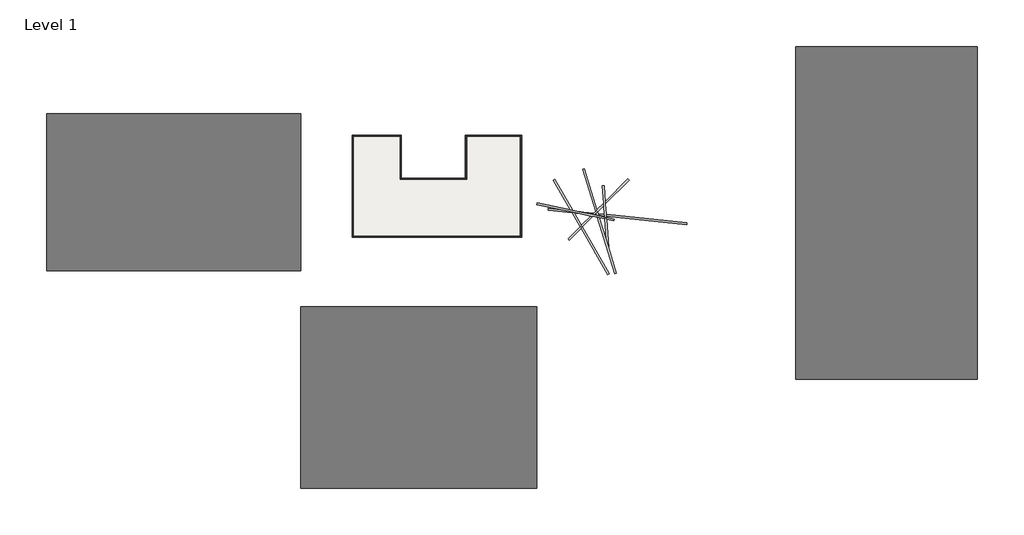
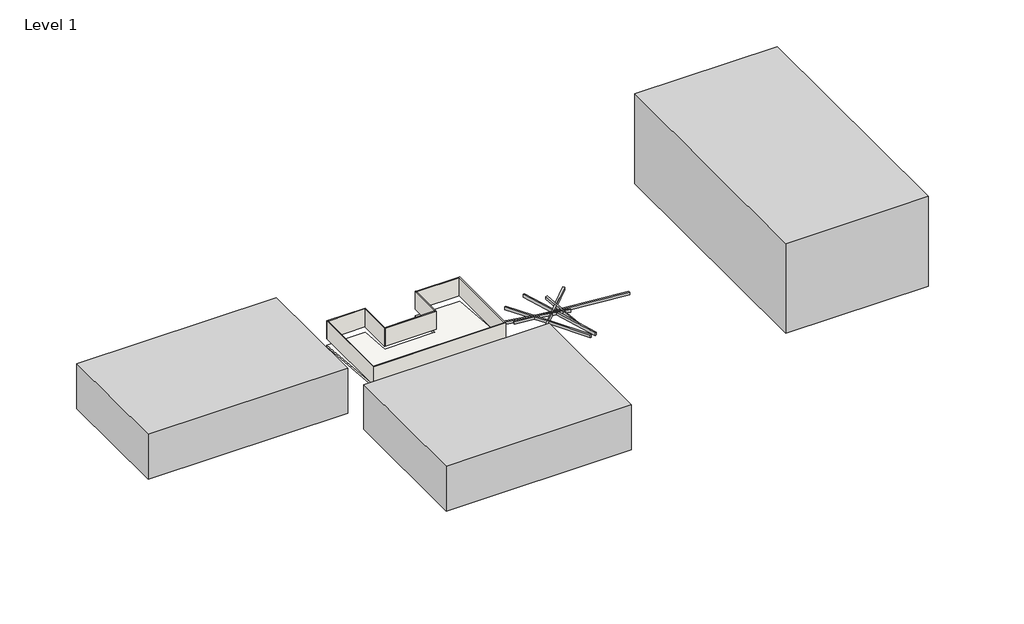
# One storey: 8 walls, 6 beams, 1 proxy, 1 slab.
"""IFC4 building model written with IfcOpenShell, lengths in millimetres."""

from ifc_helpers import new_model, si_unit, frame, origin, origin_with_axes, place, context, project, spatial, polyline, outline, extrude, faceted_brep, element, save

model = new_model("IFC4")

# Units and contexts
model_context = context("Model", 3, world=origin())
ifc_project = project(units=[si_unit("LENGTHUNIT", "METRE", prefix="MILLI")], contexts=[model_context])

# Site, building, storey
site = spatial("IfcSite", under=ifc_project)
building = spatial("IfcBuilding", under=site)
storey = spatial("IfcBuildingStorey", under=building, Name="Level 1", Elevation=0.0)

# Beams
placement = place(None, origin())
element("IfcBeam", 1, ObjectType="M_Concrete-Rectangular Beam : 300 x 600mm", at=placement, inside=storey, context=model_context, shape_type="Brep", body=[
    faceted_brep([(23275.0749275, 1168.1694607, 0.0), (23574.3441426, 1189.0964028, 0.0), (23574.3441426, 1189.0964028, -600.0), (23275.0749275, 1168.1694607, -600.0), (23478.0913387, -1735.1004802, 0.0), (23505.8198089, -2131.6360787, 0.0), (23605.6683255, -3559.5363899, 0.0), (23626.9180994, -3863.422315, 0.0), (23638.1515547, -4024.0682104, 0.0), (23659.9218408, -4335.397806, 0.0), (23902.8471924, -7809.3921842, 0.0), (24292.7609524, -9084.7426271, 0.0), (23965.19176, -4400.2849304, 0.0), (23943.4214739, -4088.9553348, 0.0), (23929.877299, -3895.26461, 0.0), (23908.6275251, -3591.3786849, 0.0), (23786.8975108, -1850.5583769, 0.0), (23759.1690405, -1454.0227784, 0.0), (24292.7609524, -9084.7426271, -600.0), (23965.19176, -4400.2849304, -600.0), (23943.4214739, -4088.9553348, -600.0), (23929.877299, -3895.26461, -600.0), (23908.6275251, -3591.3786849, -600.0), (23786.8975108, -1850.5583769, -600.0), (23759.1690405, -1454.0227784, -600.0), (23902.8471924, -7809.3921842, -600.0), (23659.9218408, -4335.397806, -600.0), (23638.1515547, -4024.0682104, -600.0), (23626.9180994, -3863.422315, -600.0), (23605.6683255, -3559.5363899, -600.0), (23505.8198089, -2131.6360787, -600.0), (23478.0913387, -1735.1004802, -600.0)], [[[0, 1, 2, 3]], [[1, 0, 4, 5, 6, 7, 8, 9, 10, 11, 12, 13, 14, 15, 16, 17]], [[2, 1, 17, 16, 15, 14, 13, 12, 11, 18, 19, 20, 21, 22, 23, 24]], [[3, 2, 24, 23, 22, 21, 20, 19, 18, 25, 26, 27, 28, 29, 30, 31]], [[0, 3, 31, 30, 29, 28, 27, 26, 25, 10, 9, 8, 7, 6, 5, 4]], [[11, 10, 25, 18]]]),
])
element("IfcBeam", 2, ObjectType="M_Concrete-Rectangular Beam : 300 x 600mm", at=placement, inside=storey, context=model_context, shape_type="Brep", body=[
    faceted_brep([(12450.0596621, -1952.6680445, 0.0), (12512.4331694, -1659.2237643, 0.0), (12512.4331694, -1659.2237643, -600.0), (12450.0596621, -1952.6680445, -600.0), (16492.4721668, -2811.9093474, 0.0), (19299.7867589, -3408.6224846, 0.0), (21365.4904585, -3847.7013604, 0.0), (21715.3826467, -3922.0732409, 0.0), (22448.2953753, -4077.8586505, 0.0), (22783.8060868, -4149.1736537, 0.0), (23659.9218408, -4335.397806, 0.0), (23638.1515547, -4024.0682104, 0.0), (22683.5207734, -3821.1551739, 0.0), (22348.0100619, -3749.8401706, 0.0), (22154.0960952, -3708.6224846, 0.0), (21968.3210977, -3669.1347899, 0.0), (21618.4289095, -3594.7629094, 0.0), (19346.7815031, -3111.9093474, 0.0), (18380.9429058, -2906.614016, 0.0), (17986.074678, -2822.6821832, 0.0), (23638.1515547, -4024.0682104, -600.0), (22683.5207734, -3821.1551739, -600.0), (22348.0100619, -3749.8401706, -600.0), (22154.0960952, -3708.6224846, -600.0), (21968.3210977, -3669.1347899, -600.0), (21618.4289095, -3594.7629094, -600.0), (19346.7815031, -3111.9093474, -600.0), (18380.9429058, -2906.614016, -600.0), (17986.074678, -2822.6821832, -600.0), (23659.9218408, -4335.397806, -600.0), (22783.8060868, -4149.1736537, -600.0), (22448.2953753, -4077.8586505, -600.0), (21715.3826467, -3922.0732409, -600.0), (21365.4904585, -3847.7013604, -600.0), (19299.7867589, -3408.6224846, -600.0), (16492.4721668, -2811.9093474, -600.0)], [[[0, 1, 2, 3]], [[1, 0, 4, 5, 6, 7, 8, 9, 10, 11, 12, 13, 14, 15, 16, 17, 18, 19]], [[2, 1, 19, 18, 17, 16, 15, 14, 13, 12, 11, 20, 21, 22, 23, 24, 25, 26, 27, 28]], [[3, 2, 28, 27, 26, 25, 24, 23, 22, 21, 20, 29, 30, 31, 32, 33, 34, 35]], [[0, 3, 35, 34, 33, 32, 31, 30, 29, 10, 9, 8, 7, 6, 5, 4]], [[11, 10, 29, 20]]]),
    faceted_brep([(25165.9784716, -4655.5200252, 0.0), (25165.9784716, -4655.5200252, -600.0), (25228.3519789, -4362.0757449, -600.0), (25228.3519789, -4362.0757449, 0.0), (23965.19176, -4400.2849304, 0.0), (23943.4214739, -4088.9553348, 0.0), (23943.4214739, -4088.9553348, -600.0), (23965.19176, -4400.2849304, -600.0)], [[[0, 1, 2, 3]], [[4, 5, 6, 7]], [[0, 3, 5, 4]], [[3, 2, 6, 5]], [[2, 1, 7, 6]], [[1, 0, 4, 7]]]),
])
element("IfcBeam", 3, ObjectType="M_Concrete-Rectangular Beam : 300 x 600mm", at=placement, inside=storey, context=model_context, shape_type="Brep", body=[
    faceted_brep([(17813.0913686, -7824.3645191, 0.0), (17600.9593342, -7612.2324847, 0.0), (17600.9593342, -7612.2324847, -600.0), (17813.0913686, -7824.3645191, -600.0), (19753.5011889, -5883.9546987, 0.0), (19973.1164312, -5664.3394565, 0.0), (21715.3826467, -3922.0732409, 0.0), (21365.4904585, -3847.7013604, 0.0), (19817.8250041, -5395.3668148, 0.0), (19598.2097619, -5614.9820571, 0.0), (21365.4904585, -3847.7013604, -600.0), (19817.8250041, -5395.3668148, -600.0), (19598.2097619, -5614.9820571, -600.0), (21715.3826467, -3922.0732409, -600.0), (19973.1164312, -5664.3394565, -600.0), (19753.5011889, -5883.9546987, -600.0)], [[[0, 1, 2, 3]], [[1, 0, 4, 5, 6, 7, 8, 9]], [[2, 1, 9, 8, 7, 10, 11, 12]], [[3, 2, 12, 11, 10, 13, 14, 15]], [[0, 3, 15, 14, 13, 6, 5, 4]], [[7, 6, 13, 10]]]),
    faceted_brep([(27712.5863052, 2075.1304175, 0.0), (27712.5863052, 2075.1304175, -600.0), (27500.4542708, 2287.2624519, -600.0), (27500.4542708, 2287.2624519, 0.0), (23786.8975108, -1850.5583769, 0.0), (23759.1690405, -1454.0227784, 0.0), (23759.1690405, -1454.0227784, -600.0), (23786.8975108, -1850.5583769, -600.0)], [[[0, 1, 2, 3]], [[4, 5, 6, 7]], [[0, 3, 5, 4]], [[3, 2, 6, 5]], [[2, 1, 7, 6]], [[1, 0, 4, 7]]]),
    faceted_brep([(23478.0913387, -1735.1004802, 0.0), (23505.8198089, -2131.6360787, 0.0), (23505.8198089, -2131.6360787, -600.0), (23478.0913387, -1735.1004802, -600.0), (21968.3210977, -3669.1347899, 0.0), (21618.4289095, -3594.7629094, 0.0), (21618.4289095, -3594.7629094, -600.0), (21968.3210977, -3669.1347899, -600.0), (22381.1258552, -2832.0659638, 0.0), (22140.8714663, -3072.3203527, 0.0), (21839.3074392, -3373.8843798, 0.0), (22223.2206079, -3414.2352798, 0.0), (22240.2108972, -3397.2449905, 0.0), (22480.4652861, -3156.9906016, 0.0), (22381.1258552, -2832.0659638, -600.0), (22140.8714663, -3072.3203527, -600.0), (21839.3074392, -3373.8843798, -600.0), (22480.4652861, -3156.9906016, -600.0), (22240.2108972, -3397.2449905, -600.0), (22223.2206079, -3414.2352798, -600.0)], [[[0, 1, 2, 3]], [[4, 5, 6, 7]], [[1, 0, 8, 9, 10, 5, 4, 11, 12, 13]], [[0, 3, 14, 15, 16, 6, 5, 10, 9, 8]], [[3, 2, 17, 18, 19, 7, 6, 16, 15, 14]], [[2, 1, 13, 12, 11, 4, 7, 19, 18, 17]]]),
])
element("IfcBeam", 4, ObjectType="M_Concrete-Rectangular Beam : 300 x 600mm", at=placement, inside=storey, context=model_context, shape_type="Brep", body=[
    faceted_brep([(25575.5456711, -13280.5423831, 0.0), (25288.6542443, -13368.2538946, 0.0), (25288.6542443, -13368.2538946, -600.0), (25575.5456711, -13280.5423831, -600.0), (24292.7609524, -9084.7426271, 0.0), (23902.8471924, -7809.3921842, 0.0), (22783.8060868, -4149.1736537, 0.0), (22448.2953753, -4077.8586505, 0.0), (22448.2953753, -4077.8586505, -600.0), (22783.8060868, -4149.1736537, -600.0), (23902.8471924, -7809.3921842, -600.0), (24292.7609524, -9084.7426271, -600.0)], [[[0, 1, 2, 3]], [[1, 0, 4, 5, 6, 7]], [[2, 1, 7, 8]], [[3, 2, 8, 9, 10, 11]], [[0, 3, 11, 10, 9, 6, 5, 4]], [[7, 6, 9, 8]]]),
    faceted_brep([(20312.8549861, 3932.9432242, 0.0), (20312.8549861, 3932.9432242, -600.0), (20025.9635593, 3845.2317128, -600.0), (20025.9635593, 3845.2317128, 0.0), (22381.1258552, -2832.0659638, 0.0), (22140.8714663, -3072.3203527, 0.0), (22140.8714663, -3072.3203527, -600.0), (22381.1258552, -2832.0659638, -600.0)], [[[0, 1, 2, 3]], [[4, 5, 6, 7]], [[0, 3, 5, 4]], [[3, 2, 6, 5]], [[2, 1, 7, 6]], [[1, 0, 4, 7]]]),
    faceted_brep([(22683.5207734, -3821.1551739, 0.0), (22348.0100619, -3749.8401706, 0.0), (22348.0100619, -3749.8401706, -600.0), (22683.5207734, -3821.1551739, -600.0), (22665.5509582, -3762.3785569, 0.0), (22570.2646476, -3450.7110782, 0.0), (22480.4652861, -3156.9906016, 0.0), (22240.2108972, -3397.2449905, 0.0), (22246.1418931, -3416.6444039, 0.0), (22341.4282037, -3728.3118826, 0.0), (22240.2108972, -3397.2449905, -600.0), (22246.1418931, -3416.6444039, -600.0), (22341.4282037, -3728.3118826, -600.0), (22480.4652861, -3156.9906016, -600.0), (22570.2646476, -3450.7110782, -600.0), (22665.5509582, -3762.3785569, -600.0)], [[[0, 1, 2, 3]], [[1, 0, 4, 5, 6, 7, 8, 9]], [[2, 1, 9, 8, 7, 10, 11, 12]], [[3, 2, 12, 11, 10, 13, 14, 15]], [[0, 3, 15, 14, 13, 6, 5, 4]], [[7, 6, 13, 10]]]),
])
element("IfcBeam", 5, ObjectType="M_Concrete-Rectangular Beam : 300 x 600mm", at=placement, inside=storey, context=model_context, shape_type="Brep", body=[
    faceted_brep([(37213.5017673, -4989.7773175, 0.0), (37182.1432283, -5288.1338861, 0.0), (37182.1432283, -5288.1338861, -600.0), (37213.5017673, -4989.7773175, -600.0), (23908.6275251, -3591.3786849, 0.0), (23929.877299, -3895.26461, 0.0), (23929.877299, -3895.26461, -600.0), (23908.6275251, -3591.3786849, -600.0)], [[[0, 1, 2, 3]], [[1, 0, 4, 5]], [[2, 1, 5, 6]], [[3, 2, 6, 7]], [[0, 3, 7, 4]], [[5, 4, 7, 6]]]),
    faceted_brep([(14339.4981738, -2585.6226623, 0.0), (14339.4981738, -2585.6226623, -600.0), (14308.1396348, -2883.9792309, -600.0), (14308.1396348, -2883.9792309, 0.0), (16492.4721668, -2811.9093474, 0.0), (19299.7867589, -3408.6224846, 0.0), (19299.7867589, -3408.6224846, -600.0), (16492.4721668, -2811.9093474, -600.0), (18261.3532922, -3299.4787292, 0.0), (18630.1422926, -3338.2400151, 0.0), (18261.3532922, -3299.4787292, -600.0), (18630.1422926, -3338.2400151, -600.0)], [[[0, 1, 2, 3]], [[4, 5, 6, 7]], [[0, 3, 8, 9, 5, 4]], [[3, 2, 10, 11, 6, 5, 9, 8]], [[2, 1, 7, 6, 11, 10]], [[1, 0, 4, 7]]]),
    faceted_brep([(23605.6683255, -3559.5363899, 0.0), (23626.9180994, -3863.422315, 0.0), (23626.9180994, -3863.422315, -600.0), (23605.6683255, -3559.5363899, -600.0), (22570.2646476, -3450.7110782, 0.0), (22665.5509582, -3762.3785569, 0.0), (22665.5509582, -3762.3785569, -600.0), (22570.2646476, -3450.7110782, -600.0)], [[[0, 1, 2, 3]], [[1, 0, 4, 5]], [[2, 1, 5, 6]], [[3, 2, 6, 7]], [[0, 3, 7, 4]], [[5, 4, 7, 6]]]),
    faceted_brep([(19346.7815031, -3111.9093474, 0.0), (19346.7815031, -3111.9093474, -600.0), (21618.4289095, -3594.7629094, -600.0), (21618.4289095, -3594.7629094, 0.0), (21839.3074392, -3373.8843798, 0.0), (21839.3074392, -3373.8843798, -600.0)], [[[0, 1, 2, 3]], [[4, 3, 2, 5]], [[4, 0, 3]], [[2, 1, 5]], [[1, 0, 4, 5]]]),
    faceted_brep([(21968.3210977, -3669.1347899, 0.0), (22223.2206079, -3414.2352798, 0.0), (22223.2206079, -3414.2352798, -600.0), (21968.3210977, -3669.1347899, -600.0), (22154.0960952, -3708.6224846, -600.0), (22154.0960952, -3708.6224846, 0.0), (22246.1418931, -3416.6444039, 0.0), (22341.4282037, -3728.3118826, 0.0), (22341.4282037, -3728.3118826, -600.0), (22246.1418931, -3416.6444039, -600.0)], [[[0, 1, 2, 3]], [[4, 5, 0, 3]], [[6, 7, 8, 9]], [[0, 5, 7, 6, 1]], [[5, 4, 8, 7]], [[4, 3, 2, 9, 8]], [[2, 1, 6, 9]]]),
])
element("IfcBeam", 6, ObjectType="M_Concrete-Rectangular Beam : 300 x 600mm", at=placement, inside=storey, context=model_context, shape_type="SweptSolid", body=[
    extrude(outline(polyline([(24428.7564122, -13381.7342838), (24168.948791, -13531.7342838), (19753.5011889, -5883.9546987), (19973.1164312, -5664.3394565), (24428.7564122, -13381.7342838)])), frame((0.0, 0.0, -600.0), z_axis=(0.0, 0.0, 1.0), x_axis=(1.0, 0.0, 0.0)), (0.0, 0.0, 1.0), 600.0),
    extrude(outline(polyline([(15168.948791, 2056.7229844), (15428.7564122, 2206.7229844), (18380.9429058, -2906.614016), (17986.074678, -2822.6821832), (15168.948791, 2056.7229844)])), frame((0.0, 0.0, -600.0), z_axis=(0.0, 0.0, 1.0), x_axis=(1.0, 0.0, 0.0)), (0.0, 0.0, 1.0), 600.0),
    extrude(outline(polyline([(19817.8250041, -5395.3668148), (19598.2097619, -5614.9820571), (18261.3532922, -3299.4787292), (18630.1422926, -3338.2400151), (19817.8250041, -5395.3668148)])), frame((0.0, 0.0, -600.0), z_axis=(0.0, 0.0, 1.0), x_axis=(1.0, 0.0, 0.0)), (0.0, 0.0, 1.0), 600.0),
])

# Proxy
element("IfcBuildingElementProxy", 7, Name="Mass 1 : Mass 1", ObjectType="Mass 1 : Mass 1", at=placement, inside=storey, context=model_context, shape_type="SweptSolid", body=[
    extrude(outline(polyline([(85281.541237, -30832.9283466), (55281.541237, -30832.9283466), (55281.541237, 24167.0716534), (85281.541237, 24167.0716534), (85281.541237, -30832.9283466)])), origin_with_axes(), (0.0, 0.0, 1.0), 20000.0),
    extrude(outline(polyline([(12385.9998775, -18841.3028807), (12385.9998775, -48841.3028807), (-26614.0001225, -48841.3028807), (-26614.0001225, -18841.3028807), (12385.9998775, -18841.3028807)])), origin_with_axes(), (0.0, 0.0, 1.0), 10000.0),
    extrude(outline(polyline([(-68614.0001225, 13088.4886322), (-26614.0001225, 13088.4886322), (-26614.0001225, -12911.5113678), (-68614.0001225, -12911.5113678), (-68614.0001225, 13088.4886322)])), origin_with_axes(), (0.0, 0.0, 1.0), 10000.0),
])

# Slab
element("IfcSlab", 8, ObjectType="Generic Floor - 400mm", at=placement, inside=storey, context=model_context, shape_type="Brep", body=[
    faceted_brep([(-9981.2219475, 9504.7039339, -1809.7198193), (-9981.2219475, 2393.7709904, -1217.142074), (618.7780525, 2393.7709904, -1217.142074), (618.7780525, 9504.7039339, -1809.7198193), (9919.5632793, 9504.7039339, -1809.7198193), (9919.5632793, -7395.2960661, -401.386486), (-18080.4367207, -7395.2960661, -401.386486), (-18080.4367207, 9504.7039339, -1809.7198193), (-9981.2219475, 9504.7039339, -1408.3333333), (-18080.4367207, 9504.7039339, -1408.3333333), (-18080.4367207, -7395.2960661, 0.0), (9919.5632793, -7395.2960661, 0.0), (9919.5632793, 9504.7039339, -1408.3333333), (618.7780525, 9504.7039339, -1408.3333333), (618.7780525, 2393.7709904, -815.755588), (-9981.2219475, 2393.7709904, -815.755588)], [[[0, 1, 2, 3, 4, 5, 6, 7]], [[8, 9, 10, 11, 12, 13, 14, 15]], [[1, 0, 8, 15]], [[2, 1, 15, 14]], [[3, 2, 14, 13]], [[4, 3, 13, 12]], [[5, 4, 12, 11]], [[6, 5, 11, 10]], [[7, 6, 10, 9]], [[0, 7, 9, 8]]]),
])

# Walls
element("IfcWall", 9, ObjectType="Generic - 200mm", at=placement, inside=storey, context=model_context, shape_type="Brep", body=[
    faceted_brep([(-18080.4367207, 9304.7039339, 0.0), (-17880.4367207, 9304.7039339, 0.0), (-10181.2219475, 9304.7039339, 0.0), (-9981.2219475, 9304.7039339, 0.0), (-9981.2219475, 9304.7039339, 4000.0), (-10181.2219475, 9304.7039339, 4000.0), (-17880.4367207, 9304.7039339, 4000.0), (-18080.4367207, 9304.7039339, 4000.0), (-18080.4367207, 9504.7039339, 0.0), (-18080.4367207, 9504.7039339, 4000.0), (-9981.2219475, 9504.7039339, 4000.0), (-9981.2219475, 9504.7039339, 0.0)], [[[0, 1, 2, 3, 4, 5, 6, 7]], [[8, 9, 10, 11]], [[3, 2, 1, 0, 8, 11]], [[7, 6, 5, 4, 10, 9]], [[0, 7, 9, 8]], [[4, 3, 11, 10]]]),
])
element("IfcWall", 10, ObjectType="Generic - 200mm", at=placement, inside=storey, context=model_context, shape_type="Brep", body=[
    faceted_brep([(-17880.4367207, -7395.2960661, 0.0), (-17880.4367207, -7195.2960661, 0.0), (-17880.4367207, 9304.7039339, 0.0), (-17880.4367207, 9304.7039339, 4000.0), (-17880.4367207, -7195.2960661, 4000.0), (-17880.4367207, -7395.2960661, 4000.0), (-18080.4367207, -7395.2960661, 0.0), (-18080.4367207, -7395.2960661, 4000.0), (-18080.4367207, 9304.7039339, 4000.0), (-18080.4367207, 9304.7039339, 0.0)], [[[0, 1, 2, 3, 4, 5]], [[6, 7, 8, 9]], [[2, 1, 0, 6, 9]], [[5, 4, 3, 8, 7]], [[0, 5, 7, 6]], [[3, 2, 9, 8]]]),
])
element("IfcWall", 11, ObjectType="Generic - 200mm", at=placement, inside=storey, context=model_context, shape_type="Brep", body=[
    faceted_brep([(9919.5632793, -7195.2960661, 0.0), (9719.5632793, -7195.2960661, 0.0), (-17880.4367207, -7195.2960661, 0.0), (-17880.4367207, -7195.2960661, 4000.0), (9719.5632793, -7195.2960661, 4000.0), (9919.5632793, -7195.2960661, 4000.0), (9919.5632793, -7395.2960661, 0.0), (9919.5632793, -7395.2960661, 4000.0), (-17880.4367207, -7395.2960661, 4000.0), (-17880.4367207, -7395.2960661, 0.0)], [[[0, 1, 2, 3, 4, 5]], [[6, 7, 8, 9]], [[2, 1, 0, 6, 9]], [[5, 4, 3, 8, 7]], [[0, 5, 7, 6]], [[3, 2, 9, 8]]]),
])
element("IfcWall", 12, ObjectType="Generic - 200mm", at=placement, inside=storey, context=model_context, shape_type="Brep", body=[
    faceted_brep([(9719.5632793, 9504.7039339, 0.0), (9719.5632793, 9304.7039339, 0.0), (9719.5632793, -7195.2960661, 0.0), (9719.5632793, -7195.2960661, 4000.0), (9719.5632793, 9304.7039339, 4000.0), (9719.5632793, 9504.7039339, 4000.0), (9919.5632793, 9504.7039339, 0.0), (9919.5632793, 9504.7039339, 4000.0), (9919.5632793, -7195.2960661, 4000.0), (9919.5632793, -7195.2960661, 0.0)], [[[0, 1, 2, 3, 4, 5]], [[6, 7, 8, 9]], [[2, 1, 0, 6, 9]], [[5, 4, 3, 8, 7]], [[0, 5, 7, 6]], [[3, 2, 9, 8]]]),
])
element("IfcWall", 13, ObjectType="Generic - 200mm", at=placement, inside=storey, context=model_context, shape_type="Brep", body=[
    faceted_brep([(-9981.2219475, 2193.7709904, 0.0), (-9981.2219475, 2393.7709904, 0.0), (-9981.2219475, 9304.7039339, 0.0), (-9981.2219475, 9304.7039339, 4000.0), (-9981.2219475, 2393.7709904, 4000.0), (-9981.2219475, 2193.7709904, 4000.0), (-10181.2219475, 2193.7709904, 0.0), (-10181.2219475, 2193.7709904, 4000.0), (-10181.2219475, 9304.7039339, 4000.0), (-10181.2219475, 9304.7039339, 0.0)], [[[0, 1, 2, 3, 4, 5]], [[6, 7, 8, 9]], [[2, 1, 0, 6, 9]], [[5, 4, 3, 8, 7]], [[0, 5, 7, 6]], [[3, 2, 9, 8]]]),
])
element("IfcWall", 14, ObjectType="Generic - 200mm", at=placement, inside=storey, context=model_context, shape_type="Brep", body=[
    faceted_brep([(818.7780525, 2393.7709904, 0.0), (618.7780525, 2393.7709904, 0.0), (-9981.2219475, 2393.7709904, 0.0), (-9981.2219475, 2393.7709904, 4000.0), (618.7780525, 2393.7709904, 4000.0), (818.7780525, 2393.7709904, 4000.0), (818.7780525, 2193.7709904, 0.0), (818.7780525, 2193.7709904, 4000.0), (-9981.2219475, 2193.7709904, 4000.0), (-9981.2219475, 2193.7709904, 0.0)], [[[0, 1, 2, 3, 4, 5]], [[6, 7, 8, 9]], [[2, 1, 0, 6, 9]], [[5, 4, 3, 8, 7]], [[0, 5, 7, 6]], [[3, 2, 9, 8]]]),
])
element("IfcWall", 15, ObjectType="Generic - 200mm", at=placement, inside=storey, context=model_context, shape_type="Brep", body=[
    faceted_brep([(618.7780525, 9504.7039339, 0.0), (618.7780525, 2393.7709904, 0.0), (618.7780525, 2393.7709904, 4000.0), (618.7780525, 9504.7039339, 4000.0), (818.7780525, 9504.7039339, 0.0), (818.7780525, 9504.7039339, 4000.0), (818.7780525, 9304.7039339, 4000.0), (818.7780525, 2393.7709904, 4000.0), (818.7780525, 2393.7709904, 0.0), (818.7780525, 9304.7039339, 0.0)], [[[0, 1, 2, 3]], [[4, 5, 6, 7, 8, 9]], [[1, 0, 4, 9, 8]], [[3, 2, 7, 6, 5]], [[2, 1, 8, 7]], [[0, 3, 5, 4]]]),
])
element("IfcWall", 16, ObjectType="Generic - 200mm", at=placement, inside=storey, context=model_context, shape_type="SweptSolid", body=[
    extrude(outline(polyline([(9719.5632793, 9304.7039339), (818.7780525, 9304.7039339), (818.7780525, 9504.7039339), (9719.5632793, 9504.7039339), (9719.5632793, 9304.7039339)])), origin_with_axes(), (0.0, 0.0, 1.0), 4000.0),
])

save(model, "model.ifc")

# Revit data of these elements
# Project information
#   Project Issue Date = "Issue Date"
#   Project Status = "Project  Status"
#   Client Name = "Owner"
#   Project Address = "## Street\nCity, State  Zip"
#   Project Name = "Project Name"
#   Project Number = "0001"
# Type "M_Concrete-Rectangular Beam : 300 x 600mm"
#   Length [instance default] = 1524 mm
#   b = 300 mm
#   h = 600 mm
#   Structural Material [instance default] = Concrete, Cast-in-Place gray
#   Assembly Code = ""
# Type "Generic Floor - 400mm"
#   Function = 0
#   Layers, outside or top first: 400 mm no material (function 1)
# Type "Generic - 200mm"
#   Layers, outside or top first: 200 mm no material (function 1)
# Element 1 (IfcBeam, "M_Concrete-Rectangular Beam : 300 x 600mm")
#   Comments = "1.737"
#   test_volume = 1.737 m³
#   Phase Created = New Construction
#   Materials on its faces: "Concrete, Cast-in-Place gray"
# Element 2 (IfcBeam, "M_Concrete-Rectangular Beam : 300 x 600mm")
#   Comments = "2.284"
#   test_volume = 2.284 m³
#   Phase Created = New Construction
#   Materials on its faces: "Concrete, Cast-in-Place gray"
# Element 3 (IfcBeam, "M_Concrete-Rectangular Beam : 300 x 600mm")
#   Comments = "2.384"
#   test_volume = 2.384 m³
#   Phase Created = New Construction
#   Materials on its faces: "Concrete, Cast-in-Place gray"
# Element 4 (IfcBeam, "M_Concrete-Rectangular Beam : 300 x 600mm")
#   Comments = "3.117"
#   test_volume = 3.11701 m³
#   Phase Created = New Construction
#   Materials on its faces: "Concrete, Cast-in-Place gray"
# Element 5 (IfcBeam, "M_Concrete-Rectangular Beam : 300 x 600mm")
#   Comments = "3.449"
#   test_volume = 3.44901 m³
#   Phase Created = New Construction
#   Materials on its faces: "Concrete, Cast-in-Place gray"
# Element 6 (IfcBeam, "M_Concrete-Rectangular Beam : 300 x 600mm")
#   Comments = "3.090"
#   test_volume = 3.09001 m³
#   Phase Created = New Construction
#   Materials on its faces: "Concrete, Cast-in-Place gray"
# Element 7 (IfcBuildingElementProxy, "Mass 1 : Mass 1")
#   Phase Created = New Construction
#   Materials on its faces: "Default Form"
# Element 8 (IfcSlab, "Generic Floor - 400mm")
#   Comments = "0"
#   Height Offset From Level = 0 mm
#   test_length = 104022 mm
#   test_slope = 0.0830777 (stored number, unit not read)
#   test_int = 0
#   Phase Created = New Construction
#   Materials on its faces: "Default Roof"
# Element 9 (IfcWall, "Generic - 200mm")
#   Top Offset = 0 mm
#   Base Offset = 0 mm
#   Unconnected Height = 4000 mm
#   wall height = 4000 mm
#   test_area = 32.397 m²
#   Phase Created = New Construction
#   Base Constraint = Level 1
#   Top Constraint = Level 2
#   Materials on its faces: "Default Wall"
# Elements 10, 12 (IfcWall, "Generic - 200mm")
#   Top Offset = 0 mm
#   Base Offset = 0 mm
#   Unconnected Height = 4000 mm
#   wall height = 4000 mm
#   test_area = 66.800 m²
#   Phase Created = New Construction
#   Base Constraint = Level 1
#   Top Constraint = Level 2
#   Materials on its faces: "Default Wall"
# Element 11 (IfcWall, "Generic - 200mm")
#   Top Offset = 0 mm
#   Base Offset = 0 mm
#   Unconnected Height = 4000 mm
#   wall height = 4000 mm
#   test_area = 111.200 m²
#   Phase Created = New Construction
#   Base Constraint = Level 1
#   Top Constraint = Level 2
#   Materials on its faces: "Default Wall"
# Elements 13, 15 (IfcWall, "Generic - 200mm")
#   Top Offset = 0 mm
#   Base Offset = 0 mm
#   Unconnected Height = 4000 mm
#   wall height = 4000 mm
#   test_area = 28.444 m²
#   Phase Created = New Construction
#   Base Constraint = Level 1
#   Top Constraint = Level 2
#   Materials on its faces: "Default Wall"
# Element 14 (IfcWall, "Generic - 200mm")
#   Top Offset = 0 mm
#   Base Offset = 0 mm
#   Unconnected Height = 4000 mm
#   wall height = 4000 mm
#   test_area = 43.200 m²
#   Phase Created = New Construction
#   Base Constraint = Level 1
#   Top Constraint = Level 2
#   Materials on its faces: "Default Wall"
# Element 16 (IfcWall, "Generic - 200mm")
#   Top Offset = 0 mm
#   Base Offset = 0 mm
#   Unconnected Height = 4000 mm
#   wall height = 4000 mm
#   test_area = 35.603 m²
#   Phase Created = New Construction
#   Base Constraint = Level 1
#   Top Constraint = Level 2
#   Materials on its faces: "Default Wall"
# Materials
#   "Concrete, Cast-in-Place gray": class "Concrete", colour RGB 192 192 192, transparency 0, Description = "Cast-in-place concrete", Cost = 0
#   "Default Form": class "Generic", colour RGB 185 189 196, transparency 0.5, Cost = 0
#   "Default Roof": class "Miscellaneous", colour RGB 88 101 114, transparency 0, Cost = 0
#   "Default Wall": class "Miscellaneous", colour RGB 128 128 128, transparency 0, Cost = 0
